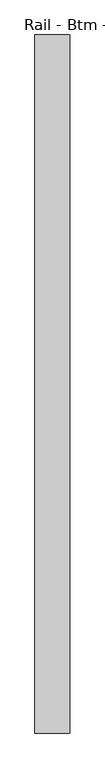
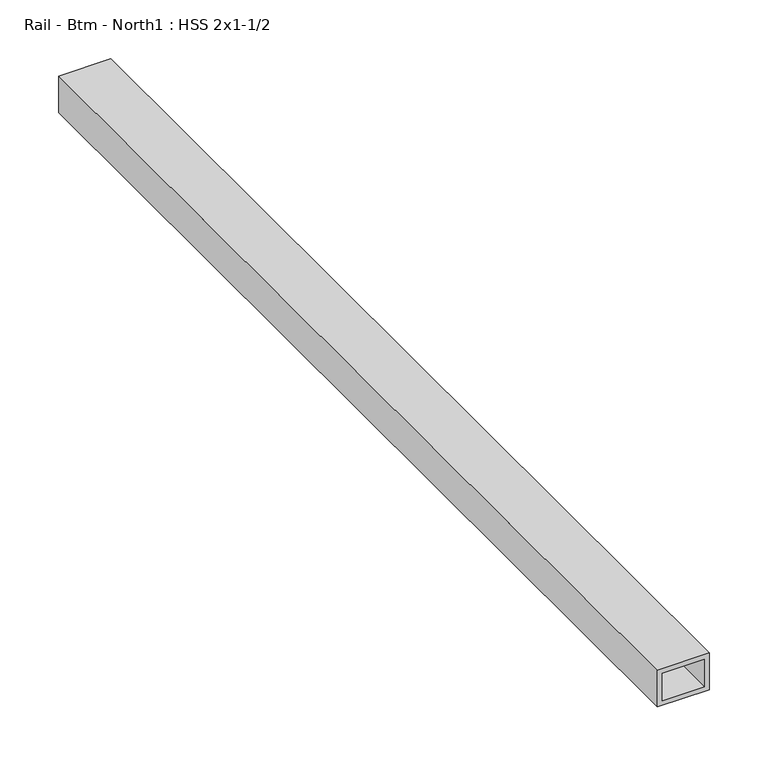
"""IFC4 building model written with IfcOpenShell, lengths in millimetres: proxy geometry, Rail - Btm - North1 : HSS 2x1-1/2."""

from ifc_helpers import new_model, si_unit, frame, origin, place, context, project, spatial, polyline, outline, extrude, source, transform, mapped, element, save


def rail_btm_north1_hss_2x1_1_2_782f6166(model_context):
    return source(origin(), model_context, "Body", "SweptSolid", [
        extrude(outline(polyline([(50.8, 587416.6934739), (88.9, 587416.6934739), (88.9, 587365.8934739), (50.8, 587365.8934739), (50.8, 587416.6934739)]), holes=[polyline([(84.1375, 587411.9309739), (55.5625, 587411.9309739), (55.5625, 587370.6559739), (84.1375, 587370.6559739), (84.1375, 587411.9309739)])]), frame((0.0, -535163.4663841, 0.0), z_axis=(0.0, 1.0, 0.0), x_axis=(0.0, 0.0, 1.0)), (0.0, 0.0, 1.0), 1016.0),
    ])


if __name__ == "__main__":
    model = new_model("IFC4")
    model_context = context("Model", 3, world=origin())
    ifc_project = project(units=[si_unit("LENGTHUNIT", "METRE", prefix="MILLI")], contexts=[model_context])
    site = spatial("IfcSite", under=ifc_project)
    building = spatial("IfcBuilding", under=site)
    placement = place(None, origin())
    rail_btm_north1_hss_2x1_1_2_shape = rail_btm_north1_hss_2x1_1_2_782f6166(model_context)
    element("IfcBuildingElementProxy", 1, Name="Rail - Btm - North1 : HSS 2x1-1/2", ObjectType="Rail - Btm - North1 : HSS 2x1-1/2", at=placement, inside=building, context=model_context, shape_type="MappedRepresentation", body=[
        mapped(rail_btm_north1_hss_2x1_1_2_shape, transform((0.0, 0.0, 0.0), x_axis=(1.0, 0.0, 0.0), y_axis=(0.0, 1.0, 0.0), z_axis=(0.0, 0.0, 1.0))),
    ])
    save(model, "model.ifc")

# Revit data of these elements
# Element 1 (IfcBuildingElementProxy, "Rail - Btm - North1 : HSS 2x1-1/2")
#   Materials on its faces: "1-1/2\"X2\" GALV. STL HSS TUBING"
# Materials
#   "1-1/2\"X2\" GALV. STL HSS TUBING": class "Generic", colour RGB 211 211 207, transparency 0, Cost = 0
